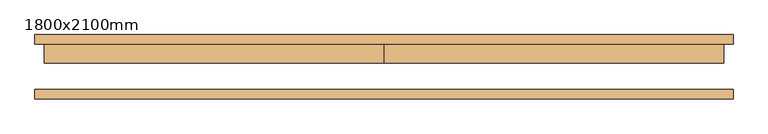
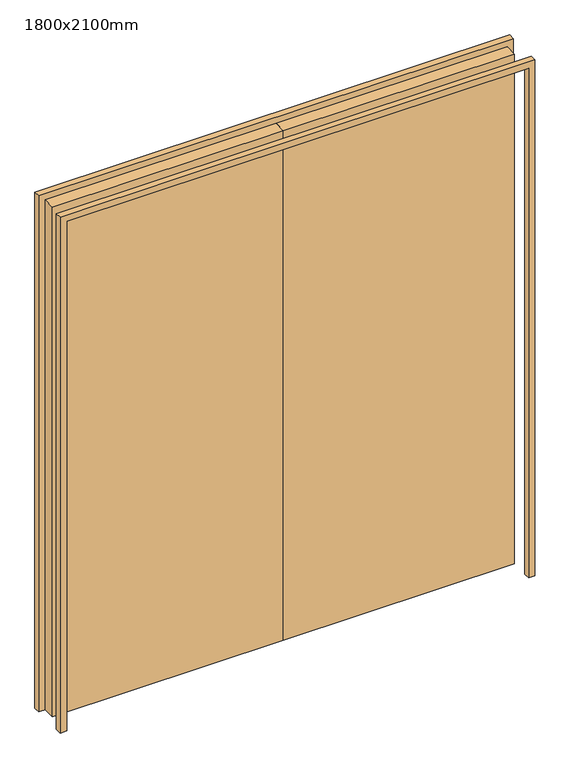
"""IFC4 building model written with IfcOpenShell, lengths in millimetres: door geometry, WWm-DoubleSolid-Flush : 1800x2100mm."""

from ifc_helpers import new_model, si_unit, frame, origin, origin_with_axes, place, context, project, spatial, polyline, outline, extrude, source, transform, mapped, element, save


def door_1800x2100mm_2ea8d6ce(model_context):
    return source(origin(), model_context, "Body", "SweptSolid", [
        extrude(outline(polyline([(0.0, 60.0), (900.0, 60.0), (900.0, 10.0), (0.0, 10.0), (0.0, 60.0)])), origin_with_axes(), (0.0, 0.0, 1.0), 2100.0),
        extrude(outline(polyline([(-900.0, 60.0), (0.0, 60.0), (0.0, 10.0), (-900.0, 10.0), (-900.0, 60.0)])), origin_with_axes(), (0.0, 0.0, 1.0), 2100.0),
        extrude(outline(polyline([(2100.0, -900.0), (2100.0, 900.0), (0.0, 900.0), (0.0, 925.0), (2125.0, 925.0), (2125.0, -925.0), (0.0, -925.0), (0.0, -900.0), (2100.0, -900.0)])), frame((0.0, -85.0, 0.0), z_axis=(0.0, 1.0, 0.0), x_axis=(0.0, 0.0, 1.0)), (0.0, 0.0, 1.0), 25.0),
        extrude(outline(polyline([(2100.0, -900.0), (2100.0, 900.0), (0.0, 900.0), (0.0, 925.0), (2125.0, 925.0), (2125.0, -925.0), (0.0, -925.0), (0.0, -900.0), (2100.0, -900.0)])), frame((0.0, 60.0, 0.0), z_axis=(0.0, 1.0, 0.0), x_axis=(0.0, 0.0, 1.0)), (0.0, 0.0, 1.0), 25.0),
    ])


if __name__ == "__main__":
    model = new_model("IFC4")
    model_context = context("Model", 3, world=origin())
    ifc_project = project(units=[si_unit("LENGTHUNIT", "METRE", prefix="MILLI")], contexts=[model_context])
    site = spatial("IfcSite", under=ifc_project)
    building = spatial("IfcBuilding", under=site)
    placement = place(None, origin())
    door_1800x2100mm_shape = door_1800x2100mm_2ea8d6ce(model_context)
    element("IfcDoor", 1, ObjectType="WWm-DoubleSolid-Flush : 1800x2100mm", at=placement, inside=building, context=model_context, shape_type="MappedRepresentation", body=[
        mapped(door_1800x2100mm_shape, transform((0.0, 0.0, 0.0), x_axis=(1.0, 0.0, 0.0), y_axis=(0.0, 1.0, 0.0), z_axis=(0.0, 0.0, 1.0))),
    ])
    save(model, "model.ifc")

# Revit data of these elements
# Type "WWm-DoubleSolid-Flush : 1800x2100mm"
#   Type Mark = "EX1-44"
#   Construction Type Id = "MDOOR"
#   Assembly Code = "C1020"
#   Analytic Construction = "Metal"
#   Thickness = 50 mm
#   Thermal Resistance (R) = 0.270117 (m²·K)/W
#   Heat Transfer Coefficient (U) = 3.7021 W/(m²·K)
#   Height = 2100 mm
#   Trim Projection Ext = 25 mm
#   Trim Projection Int = 25 mm
#   Trim Width = 25 mm
#   Width = 1800 mm
#   Not 90 Degree [instance default] = no
#   90 Degree [instance default] = yes
#   Door Material = WW-EC-RGB-White
#   Frame Material = WW-EC-RGB-White
#   Visual Light Transmittance = 0
#   Solar Heat Gain Coefficient = 0
#   Function = (empty or 0)
#   Wall Closure = (empty or 0)
# Element 1 (IfcDoor, "WWm-DoubleSolid-Flush : 1800x2100mm")
#   Materials on its faces: "WW-EC-RGB-White"
# Materials
#   "WW-EC-RGB-White": class "Generic", colour RGB 255 255 255, transparency 0, Comments = "If region requests off-white, swith asset color to RGB 231-228-220", Description = "Generic Color", Cost = 0
